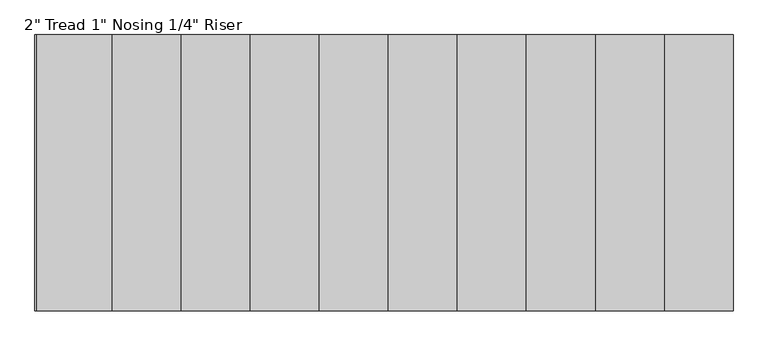
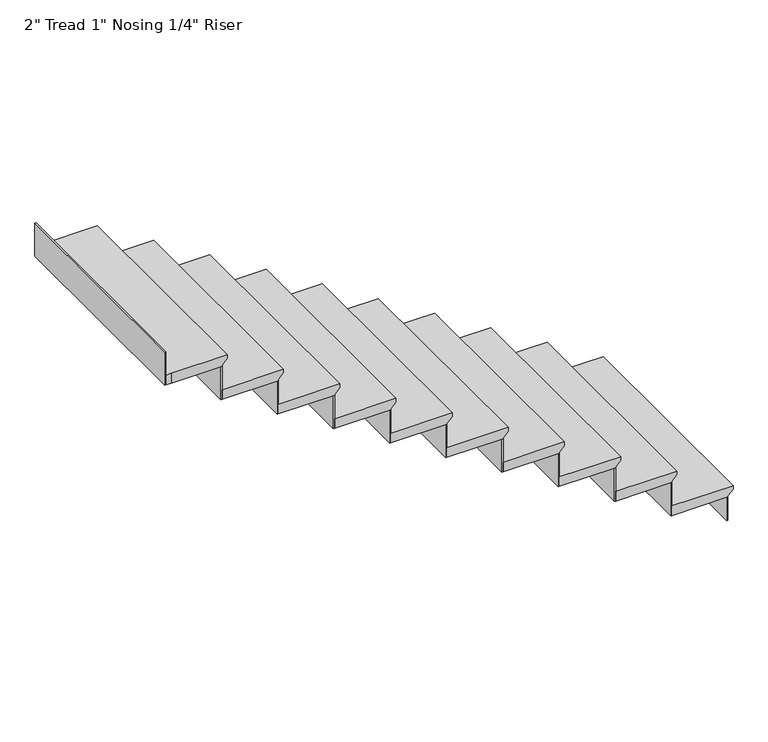
"""IFC4 building model written with IfcOpenShell, lengths in millimetres: stair flight geometry."""

import ifcopenshell
import ifcopenshell.guid

model = None  # the IFC model being written
_history = None  # IfcOwnerHistory: only IFC2X3 demands one
_inside = {}  # id of a spatial element -> (the spatial element, [elements in it])
_under = {}  # id of a project, library or spatial element -> (it, [spatial elements below it])
_declared = {}  # id of a project -> (the project, [libraries it declares])
_typed = {}  # id of a type object -> (the type object, [elements of that type])
_made_of = {}  # id of a material, layer set ... -> (it, [elements and type objects made of it])


def new_model(schema):
    """Start an empty IFC model of exactly this schema.

    Asked for "IFC4X3", IfcOpenShell would pick the latest addendum, in which some entities
    have other attributes; the version numbers below select the first issue.
    IFC2X3 requires an IfcOwnerHistory on every rooted entity: one is made here for all.
    """
    global model, _history
    if schema == "IFC4X3":
        model = ifcopenshell.file(schema_version=(4, 3, 0, 0))
    else:
        model = ifcopenshell.file(schema=schema)
    _inside.clear()
    _under.clear()
    _declared.clear()
    _typed.clear()
    _made_of.clear()
    _history = None
    if model.schema == "IFC2X3":
        org = make("IfcOrganization", Name="unknown")
        user = make(
            "IfcPersonAndOrganization",
            ThePerson=make("IfcPerson", FamilyName="unknown"),
            TheOrganization=org,
        )
        app = make(
            "IfcApplication",
            ApplicationDeveloper=org,
            Version="unknown",
            ApplicationFullName="unknown",
            ApplicationIdentifier="unknown",
        )
        _history = make(
            "IfcOwnerHistory",
            OwningUser=user,
            OwningApplication=app,
            ChangeAction="ADDED",
            CreationDate=0,
        )
    return model


def make(cls, **values):
    """One entity of the class cls with the attributes given. An attribute that is None is left unset."""
    return model.create_entity(
        cls, **{name: value for name, value in values.items() if value is not None}
    )


def rooted(cls, **values):
    """An entity with a GlobalId (a new one), such as an element, a storey or a relation."""
    return make(cls, GlobalId=ifcopenshell.guid.new(), OwnerHistory=_history, **values)


def si_unit(unit_type, name, prefix=None):
    """IfcSIUnit, for example si_unit("LENGTHUNIT", "METRE", prefix="MILLI")."""
    return make("IfcSIUnit", UnitType=unit_type, Prefix=prefix, Name=name)


def assignment(units):
    """IfcUnitAssignment: the units of a project."""
    return None if units is None else make("IfcUnitAssignment", Units=units)


def point(xyz):
    """IfcCartesianPoint."""
    return None if xyz is None else make("IfcCartesianPoint", Coordinates=xyz)


def direction(xyz):
    """IfcDirection."""
    return None if xyz is None else make("IfcDirection", DirectionRatios=xyz)


def frame(location, z_axis=None, x_axis=None):
    """IfcAxis2Placement3D, a coordinate frame: its origin and axes. An axis left out is left unset."""
    return make(
        "IfcAxis2Placement3D",
        Location=point(location),
        Axis=direction(z_axis),
        RefDirection=direction(x_axis),
    )


def origin():
    """The frame at (0, 0, 0) with its axes left unset."""
    return frame((0.0, 0.0, 0.0))


def place(relative_to, where):
    """IfcLocalPlacement: puts the frame where relative to a parent placement (None: the world)."""
    return make(
        "IfcLocalPlacement", PlacementRelTo=relative_to, RelativePlacement=where
    )


def context(
    kind, dimensions, precision=None, world=None, true_north=None, identifier=None
):
    """IfcGeometricRepresentationContext, for example the 3D "Model" context."""
    return make(
        "IfcGeometricRepresentationContext",
        ContextIdentifier=identifier,
        ContextType=kind,
        CoordinateSpaceDimension=dimensions,
        Precision=precision,
        WorldCoordinateSystem=world,
        TrueNorth=true_north,
    )


def project(units=None, contexts=None):
    """IfcProject with its units and contexts."""
    return rooted(
        "IfcProject",
        Name="project",
        RepresentationContexts=contexts,
        UnitsInContext=assignment(units),
    )


def spatial(cls, under=None, at=None, **own):
    """A site, building, storey or space (cls), placed at a placement, below another one or the project."""
    s = rooted(cls, ObjectPlacement=at, **own)
    if under is not None:
        _under.setdefault(under.id(), (under, []))[1].append(s)
    return s


def faces_of(points, faces, orient=None, outer=None):
    """IfcFace entities. A face is a list of loops; a loop is a list of indices into points, from 0.

    orient and outer hold one flag for each loop. By default every Orientation is true, the
    first loop of a face is its IfcFaceOuterBound and the others are IfcFaceBound.
    """
    made = []
    for i, loops in enumerate(faces):
        bounds = []
        for j, loop in enumerate(loops):
            is_outer = j == 0 if outer is None else outer[i][j]
            bounds.append(
                make(
                    "IfcFaceOuterBound" if is_outer else "IfcFaceBound",
                    Bound=make("IfcPolyLoop", Polygon=[points[k] for k in loop]),
                    Orientation=True if orient is None else orient[i][j],
                )
            )
        made.append(make("IfcFace", Bounds=bounds))
    return made


def faceted_brep(points, faces, orient=None, outer=None, voids=None):
    """IfcFacetedBrep: a solid bounded by flat faces; with voids (closed shells), ...WithVoids."""
    shared = [point(p) for p in points]
    hull = make("IfcClosedShell", CfsFaces=faces_of(shared, faces, orient, outer))
    if voids is None:
        return make("IfcFacetedBrep", Outer=hull)
    return make(
        "IfcFacetedBrepWithVoids",
        Outer=hull,
        Voids=[
            make(cls, CfsFaces=faces_of(shared, fs, o, b)) for cls, fs, o, b in voids
        ],
    )


def shape(context_of_items, identifier, shape_type, items):
    """IfcShapeRepresentation: the items that make up one representation, for example the "Body"."""
    return make(
        "IfcShapeRepresentation",
        ContextOfItems=context_of_items,
        RepresentationIdentifier=identifier,
        RepresentationType=shape_type,
        Items=items,
    )


def source(mapping_origin, context_of_items, identifier, shape_type, items):
    """IfcRepresentationMap: a shape defined once, which mapped items show again and again."""
    return make(
        "IfcRepresentationMap",
        MappingOrigin=mapping_origin,
        MappedRepresentation=shape(context_of_items, identifier, shape_type, items),
    )


def transform(
    local_origin,
    x_axis=None,
    y_axis=None,
    z_axis=None,
    scale=None,
    scale2=None,
    scale3=None,
    uniform=True,
):
    """IfcCartesianTransformationOperator3D, or its non-uniform kind. x_axis, y_axis, z_axis: its Axis1, 2, 3."""
    if uniform:
        return make(
            "IfcCartesianTransformationOperator3D",
            Axis1=direction(x_axis),
            Axis2=direction(y_axis),
            LocalOrigin=point(local_origin),
            Scale=scale,
            Axis3=direction(z_axis),
        )
    return make(
        "IfcCartesianTransformationOperator3DnonUniform",
        Axis1=direction(x_axis),
        Axis2=direction(y_axis),
        LocalOrigin=point(local_origin),
        Scale=scale,
        Axis3=direction(z_axis),
        Scale2=scale2,
        Scale3=scale3,
    )


def mapped(mapping_source, mapping_target):
    """IfcMappedItem: shows the shape of a source again, moved by a transform."""
    return make(
        "IfcMappedItem", MappingSource=mapping_source, MappingTarget=mapping_target
    )


def made_of(thing, what):
    """Note that an element or type object is made of a material, layer set ...; save() writes the relation."""
    if what is not None:
        _made_of.setdefault(what.id(), (what, []))[1].append(thing)
    return thing


def element(
    cls,
    number,
    at=None,
    inside=None,
    cuts=None,
    type_object=None,
    material=None,
    context=None,
    identifier="Body",
    shape_type=None,
    held_by="IfcProductDefinitionShape",
    body=None,
    shapes=None,
    **own,
):
    """One element of the class cls, such as IfcWall. Its Tag is "e" and its number.

    at: its placement. inside: the storey or other place that contains it. cuts: it is an
    opening in that element (IfcRelVoidsElement). A single representation is given by context,
    identifier, shape_type and body (its items); several are given by shapes. held_by: the class
    of the entity that holds the representations. save() writes the other relations.
    """
    e = rooted(cls, Tag="e%d" % number, ObjectPlacement=at, **own)
    if body is not None:
        shapes = [shape(context, identifier, shape_type, body)]
    if shapes is not None:
        e.Representation = make(held_by, Representations=shapes)
    if inside is not None:
        _inside.setdefault(inside.id(), (inside, []))[1].append(e)
    if cuts is not None:
        rooted(
            "IfcRelVoidsElement", RelatingBuildingElement=cuts, RelatedOpeningElement=e
        )
    if type_object is not None:
        _typed.setdefault(type_object.id(), (type_object, []))[1].append(e)
    return made_of(e, material)


def aggregate(whole, parts):
    """IfcRelAggregates: a whole, such as a stair, and the parts it consists of."""
    return rooted("IfcRelAggregates", RelatingObject=whole, RelatedObjects=parts)


def save(model, path):
    """Write the relations noted so far, then the file.

    IfcRelAggregates (storeys below a building ...), IfcRelContainedInSpatialStructure (elements
    in a storey), IfcRelDefinesByType, IfcRelAssociatesMaterial and IfcRelDeclares: one each for
    every whole, place, type object, material and project.
    """
    for whole, parts in _under.values():
        aggregate(whole, parts)
    for where, things in _inside.values():
        rooted(
            "IfcRelContainedInSpatialStructure",
            RelatedElements=things,
            RelatingStructure=where,
        )
    for kind, things in _typed.values():
        rooted("IfcRelDefinesByType", RelatedObjects=things, RelatingType=kind)
    for what, things in _made_of.values():
        rooted("IfcRelAssociatesMaterial", RelatedObjects=things, RelatingMaterial=what)
    for by, libraries in _declared.values():
        rooted("IfcRelDeclares", RelatingContext=by, RelatedDefinitions=libraries)
    model.write(path)


def stair_flight_86f709bd(model_context):
    return source(origin(), model_context, "Body", "Brep", [
        faceted_brep([(-708.6122732, 7615.1015304, 3812.7214286), (-708.6122732, 7615.1015304, 3831.7714286), (-708.6122732, 6497.5015304, 3831.7714286), (-708.6122732, 6497.5015304, 3812.7214286), (-734.0122732, 7615.1015304, 3787.3214286), (-734.0122732, 6497.5015304, 3787.3214286), (-1013.4122732, 7615.1015304, 3831.7714286), (-1013.4122732, 6497.5015304, 3831.7714286), (-734.0122732, 6497.5015304, 3780.9714286), (-1013.4122732, 6497.5015304, 3780.9714286), (-1013.4122732, 7615.1015304, 3780.9714286), (-734.0122732, 7615.1015304, 3780.9714286)], [[[0, 1, 2, 3]], [[4, 0, 3, 5]], [[2, 1, 6, 7]], [[8, 9, 10, 11]], [[2, 7, 9, 8, 5, 3]], [[8, 11, 4, 5]], [[6, 1, 0, 4, 11, 10]], [[7, 6, 10, 9]]]),
        faceted_brep([(-734.0122732, 7615.1015304, 3780.9714286), (-734.0122732, 7615.1015304, 3657.6), (-740.3622732, 7615.1015304, 3657.6), (-740.3622732, 7615.1015304, 3780.9714286), (-734.0122732, 6497.5015304, 3780.9714286), (-740.3622732, 6497.5015304, 3780.9714286), (-740.3622732, 6497.5015304, 3657.6), (-734.0122732, 6497.5015304, 3657.6)], [[[0, 1, 2, 3]], [[4, 5, 6, 7]], [[1, 0, 4, 7]], [[2, 1, 7, 6]], [[3, 2, 6, 5]], [[0, 3, 5, 4]]]),
        faceted_brep([(-1013.4122732, 7615.1015304, 3955.1428571), (-1013.4122732, 7615.1015304, 3780.9714286), (-1019.7622732, 7615.1015304, 3780.9714286), (-1019.7622732, 7615.1015304, 3955.1428571), (-1013.4122732, 6497.5015304, 3955.1428571), (-1019.7622732, 6497.5015304, 3955.1428571), (-1019.7622732, 6497.5015304, 3780.9714286), (-1013.4122732, 6497.5015304, 3780.9714286)], [[[0, 1, 2, 3]], [[4, 5, 6, 7]], [[1, 0, 4, 7]], [[2, 1, 7, 6]], [[3, 2, 6, 5]], [[0, 3, 5, 4]]]),
        faceted_brep([(-988.0122732, 6497.5015304, 4005.9428571), (-988.0122732, 7615.1015304, 4005.9428571), (-1292.8122732, 7615.1015304, 4005.9428571), (-1292.8122732, 6497.5015304, 4005.9428571), (-1013.4122732, 6497.5015304, 3955.1428571), (-1292.8122732, 6497.5015304, 3955.1428571), (-1292.8122732, 7615.1015304, 3955.1428571), (-1013.4122732, 7615.1015304, 3955.1428571), (-1013.4122732, 6497.5015304, 3961.4928571), (-988.0122732, 6497.5015304, 3986.8928571), (-1013.4122732, 7615.1015304, 3961.4928571), (-988.0122732, 7615.1015304, 3986.8928571)], [[[0, 1, 2, 3]], [[4, 5, 6, 7]], [[0, 3, 5, 4, 8, 9]], [[4, 7, 10, 8]], [[2, 1, 11, 10, 7, 6]], [[3, 2, 6, 5]], [[11, 1, 0, 9]], [[10, 11, 9, 8]]]),
        faceted_brep([(-1292.8122732, 7615.1015304, 4129.3142857), (-1292.8122732, 7615.1015304, 3955.1428571), (-1299.1622732, 7615.1015304, 3955.1428571), (-1299.1622732, 7615.1015304, 4129.3142857), (-1292.8122732, 6497.5015304, 4129.3142857), (-1299.1622732, 6497.5015304, 4129.3142857), (-1299.1622732, 6497.5015304, 3955.1428571), (-1292.8122732, 6497.5015304, 3955.1428571)], [[[0, 1, 2, 3]], [[4, 5, 6, 7]], [[1, 0, 4, 7]], [[2, 1, 7, 6]], [[3, 2, 6, 5]], [[0, 3, 5, 4]]]),
        faceted_brep([(-1267.4122732, 6497.5015304, 4180.1142857), (-1267.4122732, 7615.1015304, 4180.1142857), (-1572.2122732, 7615.1015304, 4180.1142857), (-1572.2122732, 6497.5015304, 4180.1142857), (-1292.8122732, 6497.5015304, 4129.3142857), (-1572.2122732, 6497.5015304, 4129.3142857), (-1572.2122732, 7615.1015304, 4129.3142857), (-1292.8122732, 7615.1015304, 4129.3142857), (-1292.8122732, 6497.5015304, 4135.6642857), (-1267.4122732, 6497.5015304, 4161.0642857), (-1292.8122732, 7615.1015304, 4135.6642857), (-1267.4122732, 7615.1015304, 4161.0642857)], [[[0, 1, 2, 3]], [[4, 5, 6, 7]], [[0, 3, 5, 4, 8, 9]], [[4, 7, 10, 8]], [[2, 1, 11, 10, 7, 6]], [[3, 2, 6, 5]], [[11, 1, 0, 9]], [[10, 11, 9, 8]]]),
        faceted_brep([(-1572.2122732, 7615.1015304, 4303.4857143), (-1572.2122732, 7615.1015304, 4129.3142857), (-1578.5622732, 7615.1015304, 4129.3142857), (-1578.5622732, 7615.1015304, 4303.4857143), (-1572.2122732, 6497.5015304, 4303.4857143), (-1578.5622732, 6497.5015304, 4303.4857143), (-1578.5622732, 6497.5015304, 4129.3142857), (-1572.2122732, 6497.5015304, 4129.3142857)], [[[0, 1, 2, 3]], [[4, 5, 6, 7]], [[1, 0, 4, 7]], [[2, 1, 7, 6]], [[3, 2, 6, 5]], [[0, 3, 5, 4]]]),
        faceted_brep([(-1546.8122732, 6497.5015304, 4354.2857143), (-1546.8122732, 7615.1015304, 4354.2857143), (-1851.6122732, 7615.1015304, 4354.2857143), (-1851.6122732, 6497.5015304, 4354.2857143), (-1572.2122732, 6497.5015304, 4303.4857143), (-1851.6122732, 6497.5015304, 4303.4857143), (-1851.6122732, 7615.1015304, 4303.4857143), (-1572.2122732, 7615.1015304, 4303.4857143), (-1572.2122732, 6497.5015304, 4309.8357143), (-1546.8122732, 6497.5015304, 4335.2357143), (-1572.2122732, 7615.1015304, 4309.8357143), (-1546.8122732, 7615.1015304, 4335.2357143)], [[[0, 1, 2, 3]], [[4, 5, 6, 7]], [[0, 3, 5, 4, 8, 9]], [[4, 7, 10, 8]], [[2, 1, 11, 10, 7, 6]], [[3, 2, 6, 5]], [[11, 1, 0, 9]], [[10, 11, 9, 8]]]),
        faceted_brep([(-1851.6122732, 7615.1015304, 4477.6571429), (-1851.6122732, 7615.1015304, 4303.4857143), (-1857.9622732, 7615.1015304, 4303.4857143), (-1857.9622732, 7615.1015304, 4477.6571429), (-1851.6122732, 6497.5015304, 4477.6571429), (-1857.9622732, 6497.5015304, 4477.6571429), (-1857.9622732, 6497.5015304, 4303.4857143), (-1851.6122732, 6497.5015304, 4303.4857143)], [[[0, 1, 2, 3]], [[4, 5, 6, 7]], [[1, 0, 4, 7]], [[2, 1, 7, 6]], [[3, 2, 6, 5]], [[0, 3, 5, 4]]]),
        faceted_brep([(-1826.2122732, 6497.5015304, 4528.4571429), (-1826.2122732, 7615.1015304, 4528.4571429), (-2131.0122732, 7615.1015304, 4528.4571429), (-2131.0122732, 6497.5015304, 4528.4571429), (-1851.6122732, 6497.5015304, 4477.6571429), (-2131.0122732, 6497.5015304, 4477.6571429), (-2131.0122732, 7615.1015304, 4477.6571429), (-1851.6122732, 7615.1015304, 4477.6571429), (-1851.6122732, 6497.5015304, 4484.0071429), (-1826.2122732, 6497.5015304, 4509.4071429), (-1851.6122732, 7615.1015304, 4484.0071429), (-1826.2122732, 7615.1015304, 4509.4071429)], [[[0, 1, 2, 3]], [[4, 5, 6, 7]], [[0, 3, 5, 4, 8, 9]], [[4, 7, 10, 8]], [[2, 1, 11, 10, 7, 6]], [[3, 2, 6, 5]], [[11, 1, 0, 9]], [[10, 11, 9, 8]]]),
        faceted_brep([(-2131.0122732, 7615.1015304, 4651.8285714), (-2131.0122732, 7615.1015304, 4477.6571429), (-2137.3622732, 7615.1015304, 4477.6571429), (-2137.3622732, 7615.1015304, 4651.8285714), (-2131.0122732, 6497.5015304, 4651.8285714), (-2137.3622732, 6497.5015304, 4651.8285714), (-2137.3622732, 6497.5015304, 4477.6571429), (-2131.0122732, 6497.5015304, 4477.6571429)], [[[0, 1, 2, 3]], [[4, 5, 6, 7]], [[1, 0, 4, 7]], [[2, 1, 7, 6]], [[3, 2, 6, 5]], [[0, 3, 5, 4]]]),
        faceted_brep([(-2105.6122732, 6497.5015304, 4702.6285714), (-2105.6122732, 7615.1015304, 4702.6285714), (-2410.4122732, 7615.1015304, 4702.6285714), (-2410.4122732, 6497.5015304, 4702.6285714), (-2131.0122732, 6497.5015304, 4651.8285714), (-2410.4122732, 6497.5015304, 4651.8285714), (-2410.4122732, 7615.1015304, 4651.8285714), (-2131.0122732, 7615.1015304, 4651.8285714), (-2131.0122732, 6497.5015304, 4658.1785714), (-2105.6122732, 6497.5015304, 4683.5785714), (-2131.0122732, 7615.1015304, 4658.1785714), (-2105.6122732, 7615.1015304, 4683.5785714)], [[[0, 1, 2, 3]], [[4, 5, 6, 7]], [[0, 3, 5, 4, 8, 9]], [[4, 7, 10, 8]], [[2, 1, 11, 10, 7, 6]], [[3, 2, 6, 5]], [[11, 1, 0, 9]], [[10, 11, 9, 8]]]),
        faceted_brep([(-2410.4122732, 7615.1015304, 4826.0), (-2410.4122732, 7615.1015304, 4651.8285714), (-2416.7622732, 7615.1015304, 4651.8285714), (-2416.7622732, 7615.1015304, 4826.0), (-2410.4122732, 6497.5015304, 4826.0), (-2416.7622732, 6497.5015304, 4826.0), (-2416.7622732, 6497.5015304, 4651.8285714), (-2410.4122732, 6497.5015304, 4651.8285714)], [[[0, 1, 2, 3]], [[4, 5, 6, 7]], [[1, 0, 4, 7]], [[2, 1, 7, 6]], [[3, 2, 6, 5]], [[0, 3, 5, 4]]]),
        faceted_brep([(-2385.0122732, 6497.5015304, 4876.8), (-2385.0122732, 7615.1015304, 4876.8), (-2689.8122732, 7615.1015304, 4876.8), (-2689.8122732, 6497.5015304, 4876.8), (-2410.4122732, 6497.5015304, 4826.0), (-2689.8122732, 6497.5015304, 4826.0), (-2689.8122732, 7615.1015304, 4826.0), (-2410.4122732, 7615.1015304, 4826.0), (-2410.4122732, 6497.5015304, 4832.35), (-2385.0122732, 6497.5015304, 4857.75), (-2410.4122732, 7615.1015304, 4832.35), (-2385.0122732, 7615.1015304, 4857.75)], [[[0, 1, 2, 3]], [[4, 5, 6, 7]], [[0, 3, 5, 4, 8, 9]], [[4, 7, 10, 8]], [[2, 1, 11, 10, 7, 6]], [[3, 2, 6, 5]], [[11, 1, 0, 9]], [[10, 11, 9, 8]]]),
        faceted_brep([(-2689.8122732, 7615.1015304, 5000.1714286), (-2689.8122732, 7615.1015304, 4826.0), (-2696.1622732, 7615.1015304, 4826.0), (-2696.1622732, 7615.1015304, 5000.1714286), (-2689.8122732, 6497.5015304, 5000.1714286), (-2696.1622732, 6497.5015304, 5000.1714286), (-2696.1622732, 6497.5015304, 4826.0), (-2689.8122732, 6497.5015304, 4826.0)], [[[0, 1, 2, 3]], [[4, 5, 6, 7]], [[1, 0, 4, 7]], [[2, 1, 7, 6]], [[3, 2, 6, 5]], [[0, 3, 5, 4]]]),
        faceted_brep([(-2664.4122732, 6497.5015304, 5050.9714286), (-2664.4122732, 7615.1015304, 5050.9714286), (-2969.2122732, 7615.1015304, 5050.9714286), (-2969.2122732, 6497.5015304, 5050.9714286), (-2689.8122732, 6497.5015304, 5000.1714286), (-2969.2122732, 6497.5015304, 5000.1714286), (-2969.2122732, 7615.1015304, 5000.1714286), (-2689.8122732, 7615.1015304, 5000.1714286), (-2689.8122732, 6497.5015304, 5006.5214286), (-2664.4122732, 6497.5015304, 5031.9214286), (-2689.8122732, 7615.1015304, 5006.5214286), (-2664.4122732, 7615.1015304, 5031.9214286)], [[[0, 1, 2, 3]], [[4, 5, 6, 7]], [[0, 3, 5, 4, 8, 9]], [[4, 7, 10, 8]], [[2, 1, 11, 10, 7, 6]], [[3, 2, 6, 5]], [[11, 1, 0, 9]], [[10, 11, 9, 8]]]),
        faceted_brep([(-2969.2122732, 7615.1015304, 5174.3428571), (-2969.2122732, 7615.1015304, 5000.1714286), (-2975.5622732, 7615.1015304, 5000.1714286), (-2975.5622732, 7615.1015304, 5174.3428571), (-2969.2122732, 6497.5015304, 5174.3428571), (-2975.5622732, 6497.5015304, 5174.3428571), (-2975.5622732, 6497.5015304, 5000.1714286), (-2969.2122732, 6497.5015304, 5000.1714286)], [[[0, 1, 2, 3]], [[4, 5, 6, 7]], [[1, 0, 4, 7]], [[2, 1, 7, 6]], [[3, 2, 6, 5]], [[0, 3, 5, 4]]]),
        faceted_brep([(-2943.8122732, 6497.5015304, 5225.1428571), (-2943.8122732, 7615.1015304, 5225.1428571), (-3248.6122732, 7615.1015304, 5225.1428571), (-3248.6122732, 6497.5015304, 5225.1428571), (-2969.2122732, 6497.5015304, 5174.3428571), (-3248.6122732, 6497.5015304, 5174.3428571), (-3248.6122732, 7615.1015304, 5174.3428571), (-2969.2122732, 7615.1015304, 5174.3428571), (-2969.2122732, 6497.5015304, 5180.6928571), (-2943.8122732, 6497.5015304, 5206.0928571), (-2969.2122732, 7615.1015304, 5180.6928571), (-2943.8122732, 7615.1015304, 5206.0928571)], [[[0, 1, 2, 3]], [[4, 5, 6, 7]], [[0, 3, 5, 4, 8, 9]], [[4, 7, 10, 8]], [[2, 1, 11, 10, 7, 6]], [[3, 2, 6, 5]], [[11, 1, 0, 9]], [[10, 11, 9, 8]]]),
        faceted_brep([(-3528.0122732, 7615.1015304, 5522.6857143), (-3528.0122732, 7615.1015304, 5348.5142857), (-3534.3622732, 7615.1015304, 5348.5142857), (-3534.3622732, 7615.1015304, 5522.6857143), (-3528.0122732, 6497.5015304, 5522.6857143), (-3534.3622732, 6497.5015304, 5522.6857143), (-3534.3622732, 6497.5015304, 5348.5142857), (-3528.0122732, 6497.5015304, 5348.5142857)], [[[0, 1, 2, 3]], [[4, 5, 6, 7]], [[1, 0, 4, 7]], [[2, 1, 7, 6]], [[3, 2, 6, 5]], [[0, 3, 5, 4]]]),
        faceted_brep([(-3248.6122732, 7615.1015304, 5348.5142857), (-3248.6122732, 7615.1015304, 5174.3428571), (-3254.9622732, 7615.1015304, 5174.3428571), (-3254.9622732, 7615.1015304, 5348.5142857), (-3248.6122732, 6497.5015304, 5348.5142857), (-3254.9622732, 6497.5015304, 5348.5142857), (-3254.9622732, 6497.5015304, 5174.3428571), (-3248.6122732, 6497.5015304, 5174.3428571)], [[[0, 1, 2, 3]], [[4, 5, 6, 7]], [[1, 0, 4, 7]], [[2, 1, 7, 6]], [[3, 2, 6, 5]], [[0, 3, 5, 4]]]),
        faceted_brep([(-3528.0122732, 6497.5015304, 5399.3142857), (-3502.6122732, 6497.5015304, 5399.3142857), (-3223.2122732, 6497.5015304, 5399.3142857), (-3223.2122732, 7615.1015304, 5399.3142857), (-3528.0122732, 7615.1015304, 5399.3142857), (-3502.6122732, 6497.5015304, 5348.5142857), (-3528.0122732, 6497.5015304, 5348.5142857), (-3528.0122732, 7615.1015304, 5348.5142857), (-3248.6122732, 7615.1015304, 5348.5142857), (-3248.6122732, 6497.5015304, 5348.5142857), (-3248.6122732, 6497.5015304, 5354.8642857), (-3223.2122732, 6497.5015304, 5380.2642857), (-3248.6122732, 7615.1015304, 5354.8642857), (-3223.2122732, 7615.1015304, 5380.2642857)], [[[0, 1, 2, 3, 4]], [[5, 6, 7, 8, 9]], [[1, 0, 6, 5]], [[2, 1, 5, 9, 10, 11]], [[9, 8, 12, 10]], [[4, 3, 13, 12, 8, 7]], [[0, 4, 7, 6]], [[13, 3, 2, 11]], [[12, 13, 11, 10]]]),
    ])


if __name__ == "__main__":
    model = new_model("IFC4")
    model_context = context("Model", 3, world=origin())
    ifc_project = project(units=[si_unit("LENGTHUNIT", "METRE", prefix="MILLI")], contexts=[model_context])
    site = spatial("IfcSite", under=ifc_project)
    building = spatial("IfcBuilding", under=site)
    placement = place(None, origin())
    stair_flight_shape = stair_flight_86f709bd(model_context)
    element("IfcStairFlight", 1, ObjectType="2\" Tread 1\" Nosing 1/4\" Riser", at=placement, inside=building, context=model_context, shape_type="MappedRepresentation", body=[
        mapped(stair_flight_shape, transform((0.0, 0.0, 0.0), x_axis=(1.0, 0.0, 0.0), y_axis=(0.0, 1.0, 0.0), z_axis=(0.0, 0.0, 1.0))),
    ])
    save(model, "model.ifc")
